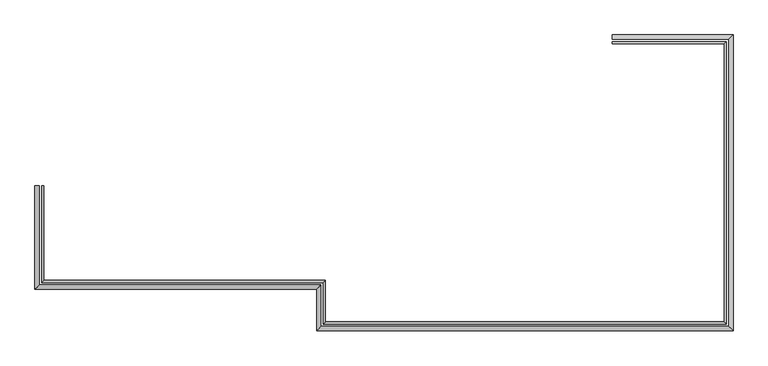
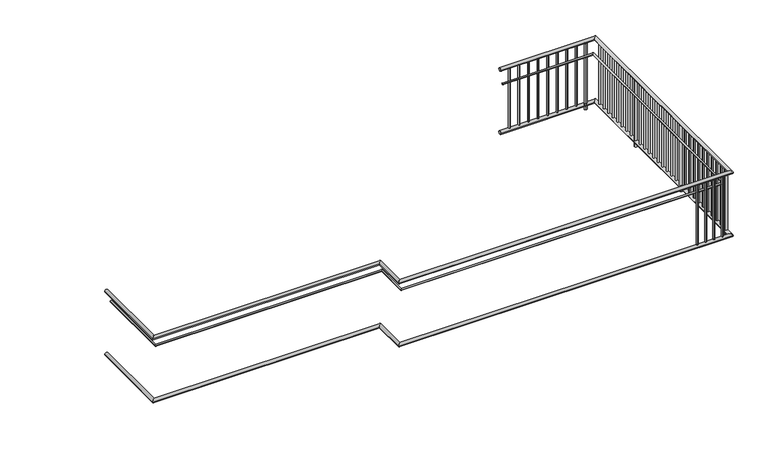
"""IFC4 building model written with IfcOpenShell, lengths in millimetres: railing geometry."""

from ifc_helpers import new_model, si_unit, point, frame, frame_2d, origin, place, context, project, spatial, circle_curve, ellipse_curve, trimmed, segment, composite_curve, outline, extrude, source, transform, mapped, element, save
from ifc_brep_helpers import plane_surface, cylinder_surface, advanced_brep


def railing_80b2a91e(model_context):
    return source(origin(), model_context, "Body", "SolidModel", [
        advanced_brep(
        [(-3300.274449, -6943.3965465, 4474.6), (-3249.474449, -6943.3965465, 4474.6), (-3249.474449, -8138.3965465, 4474.6), (-3300.274449, -8189.1965465, 4474.6), (144.725551, -8138.3965465, 4474.6), (93.925551, -8189.1965465, 4474.6), (144.725551, -8638.3965465, 4474.6), (93.925551, -8689.1965465, 4474.6), (5057.425551, -8638.3965465, 4474.6), (5108.225551, -8689.1965465, 4474.6), (5057.425551, -5178.2252792, 4474.6), (5108.225551, -5127.4252792, 4474.6), (3654.725551, -5127.4252792, 4474.6), (3654.725551, -5178.2252792, 4474.6)],
        [
            (0, 1, circle_curve(frame((-3274.874449, -6943.3965465, 4474.6), z_axis=(0.0, 1.0, 0.0), x_axis=(1.0, 0.0, 0.0)), 25.4)),
            (1, 0, circle_curve(frame((-3274.874449, -6943.3965465, 4474.6), z_axis=(0.0, 1.0, 0.0), x_axis=(1.0, 0.0, 0.0)), 25.4)),
            (1, 2),
            (2, 3, ellipse_curve(frame((-3274.874449, -8163.7965465, 4474.6), z_axis=(-0.7071067811865475, 0.7071067811865475, 0.0), x_axis=(0.7071067811865474, 0.7071067811865476, 0.0)), 35.9210245, 25.4)),
            (3, 0),
            (3, 2, ellipse_curve(frame((-3274.874449, -8163.7965465, 4474.6), z_axis=(-0.7071067811865475, 0.7071067811865475, 0.0), x_axis=(0.7071067811865474, 0.7071067811865476, 0.0)), 35.9210245, 25.4)),
            (2, 4),
            (4, 5, ellipse_curve(frame((119.325551, -8163.7965465, 4474.6), z_axis=(-0.7071067811865475, 0.7071067811865475, 0.0), x_axis=(-0.7071067811865476, -0.7071067811865474, 0.0)), 35.9210245, 25.4)),
            (5, 3),
            (5, 4, ellipse_curve(frame((119.325551, -8163.7965465, 4474.6), z_axis=(-0.7071067811865475, 0.7071067811865475, 0.0), x_axis=(-0.7071067811865476, -0.7071067811865474, 0.0)), 35.9210245, 25.4)),
            (4, 6),
            (6, 7, ellipse_curve(frame((119.325551, -8663.7965465, 4474.6), z_axis=(-0.7071067811865475, 0.7071067811865475, 0.0), x_axis=(0.7071067811865474, 0.7071067811865476, 0.0)), 35.9210245, 25.4)),
            (7, 5),
            (7, 6, ellipse_curve(frame((119.325551, -8663.7965465, 4474.6), z_axis=(-0.7071067811865475, 0.7071067811865475, 0.0), x_axis=(0.7071067811865474, 0.7071067811865476, 0.0)), 35.9210245, 25.4)),
            (6, 8),
            (8, 9, ellipse_curve(frame((5082.825551, -8663.7965465, 4474.6), z_axis=(-0.7071067811865475, -0.7071067811865475, 0.0), x_axis=(-0.7071067811865476, 0.7071067811865474, 0.0)), 35.9210245, 25.4)),
            (9, 7),
            (9, 8, ellipse_curve(frame((5082.825551, -8663.7965465, 4474.6), z_axis=(-0.7071067811865475, -0.7071067811865475, 0.0), x_axis=(-0.7071067811865476, 0.7071067811865474, 0.0)), 35.9210245, 25.4)),
            (8, 10),
            (10, 11, ellipse_curve(frame((5082.825551, -5152.8252792, 4474.6), z_axis=(0.7071067811865475, -0.7071067811865475, 0.0), x_axis=(-0.7071067811865474, -0.7071067811865476, 0.0)), 35.9210245, 25.4)),
            (11, 9),
            (11, 10, ellipse_curve(frame((5082.825551, -5152.8252792, 4474.6), z_axis=(0.7071067811865475, -0.7071067811865475, 0.0), x_axis=(-0.7071067811865474, -0.7071067811865476, 0.0)), 35.9210245, 25.4)),
            (12, 13, circle_curve(frame((3654.725551, -5152.8252792, 4474.6), z_axis=(-1.0, 0.0, 0.0), x_axis=(0.0, -1.0, 0.0)), 25.4)),
            (13, 12, circle_curve(frame((3654.725551, -5152.8252792, 4474.6), z_axis=(-1.0, 0.0, 0.0), x_axis=(0.0, -1.0, 0.0)), 25.4)),
            (10, 13),
            (12, 11),
        ],
        [
            plane_surface(frame((-3274.874449, -6943.3965465, 4500.0), z_axis=(0.0, 1.0, 0.0), x_axis=(0.0, 0.0, -1.0))),
            cylinder_surface(frame((-3274.874449, -6943.3965465, 4474.6), z_axis=(0.0, 1.0, 0.0), x_axis=(1.0, 0.0, 0.0)), 25.4),
            cylinder_surface(frame((-3274.874449, -8163.7965465, 4474.6), z_axis=(-1.0, 0.0, 0.0), x_axis=(0.0, 1.0, 0.0)), 25.4),
            cylinder_surface(frame((119.325551, -8163.7965465, 4474.6), z_axis=(0.0, 1.0, 0.0), x_axis=(1.0, 0.0, 0.0)), 25.4),
            cylinder_surface(frame((119.325551, -8663.7965465, 4474.6), z_axis=(-1.0, 0.0, 0.0), x_axis=(0.0, 1.0, 0.0)), 25.4),
            cylinder_surface(frame((5082.825551, -8663.7965465, 4474.6), z_axis=(0.0, -1.0, 0.0), x_axis=(-1.0, 0.0, 0.0)), 25.4),
            plane_surface(frame((3654.725551, -5152.8252792, 4500.0), z_axis=(-1.0, 0.0, 0.0), x_axis=(0.0, -1.0, 0.0))),
            cylinder_surface(frame((5082.825551, -5152.8252792, 4474.6), z_axis=(1.0, 0.0, 0.0), x_axis=(0.0, -1.0, 0.0)), 25.4),
        ],
        [
            (0, [[1, 2]]),
            (1, [[-2, 3, 4, 5]]),
            (1, [[-1, -5, 6, -3]]),
            (2, [[-4, 7, 8, 9]]),
            (2, [[-6, -9, 10, -7]]),
            (3, [[-8, 11, 12, 13]]),
            (3, [[-10, -13, 14, -11]]),
            (4, [[-12, 15, 16, 17]]),
            (4, [[-14, -17, 18, -15]]),
            (5, [[-16, 19, 20, 21]]),
            (5, [[-18, -21, 22, -19]]),
            (6, [[23, 24]]),
            (7, [[-20, 25, -23, 26]]),
            (7, [[-22, -26, -24, -25]]),
        ],
    ),
        advanced_brep(
        [(-3220.574449, -6943.3965465, 4287.3), (-3195.174449, -6943.3965465, 4287.3), (-3195.174449, -8084.0965465, 4287.3), (-3220.574449, -8109.4965465, 4287.3), (199.025551, -8084.0965465, 4287.3), (173.625551, -8109.4965465, 4287.3), (199.025551, -8584.0965465, 4287.3), (173.625551, -8609.4965465, 4287.3), (5003.125551, -8584.0965465, 4287.3), (5028.525551, -8609.4965465, 4287.3), (5003.125551, -5232.5252792, 4287.3), (5028.525551, -5207.1252792, 4287.3), (3654.725551, -5207.1252792, 4287.3), (3654.725551, -5232.5252792, 4287.3)],
        [
            (0, 1, circle_curve(frame((-3207.874449, -6943.3965465, 4287.3), z_axis=(0.0, 1.0, 0.0), x_axis=(1.0, 0.0, 0.0)), 12.7)),
            (1, 0, circle_curve(frame((-3207.874449, -6943.3965465, 4287.3), z_axis=(0.0, 1.0, 0.0), x_axis=(1.0, 0.0, 0.0)), 12.7)),
            (1, 2),
            (2, 3, ellipse_curve(frame((-3207.874449, -8096.7965465, 4287.3), z_axis=(-0.7071067811865475, 0.7071067811865475, 0.0), x_axis=(0.7071067811865474, 0.7071067811865476, 0.0)), 17.9605122, 12.7)),
            (3, 0),
            (3, 2, ellipse_curve(frame((-3207.874449, -8096.7965465, 4287.3), z_axis=(-0.7071067811865475, 0.7071067811865475, 0.0), x_axis=(0.7071067811865474, 0.7071067811865476, 0.0)), 17.9605122, 12.7)),
            (2, 4),
            (4, 5, ellipse_curve(frame((186.325551, -8096.7965465, 4287.3), z_axis=(-0.7071067811865475, 0.7071067811865475, 0.0), x_axis=(-0.7071067811865476, -0.7071067811865474, 0.0)), 17.9605122, 12.7)),
            (5, 3),
            (5, 4, ellipse_curve(frame((186.325551, -8096.7965465, 4287.3), z_axis=(-0.7071067811865475, 0.7071067811865475, 0.0), x_axis=(-0.7071067811865476, -0.7071067811865474, 0.0)), 17.9605122, 12.7)),
            (4, 6),
            (6, 7, ellipse_curve(frame((186.325551, -8596.7965465, 4287.3), z_axis=(-0.7071067811865475, 0.7071067811865475, 0.0), x_axis=(0.7071067811865474, 0.7071067811865476, 0.0)), 17.9605122, 12.7)),
            (7, 5),
            (7, 6, ellipse_curve(frame((186.325551, -8596.7965465, 4287.3), z_axis=(-0.7071067811865475, 0.7071067811865475, 0.0), x_axis=(0.7071067811865474, 0.7071067811865476, 0.0)), 17.9605122, 12.7)),
            (6, 8),
            (8, 9, ellipse_curve(frame((5015.825551, -8596.7965465, 4287.3), z_axis=(-0.7071067811865475, -0.7071067811865475, 0.0), x_axis=(-0.7071067811865476, 0.7071067811865474, 0.0)), 17.9605122, 12.7)),
            (9, 7),
            (9, 8, ellipse_curve(frame((5015.825551, -8596.7965465, 4287.3), z_axis=(-0.7071067811865475, -0.7071067811865475, 0.0), x_axis=(-0.7071067811865476, 0.7071067811865474, 0.0)), 17.9605122, 12.7)),
            (8, 10),
            (10, 11, ellipse_curve(frame((5015.825551, -5219.8252792, 4287.3), z_axis=(0.7071067811865475, -0.7071067811865475, 0.0), x_axis=(-0.7071067811865474, -0.7071067811865476, 0.0)), 17.9605122, 12.7)),
            (11, 9),
            (11, 10, ellipse_curve(frame((5015.825551, -5219.8252792, 4287.3), z_axis=(0.7071067811865475, -0.7071067811865475, 0.0), x_axis=(-0.7071067811865474, -0.7071067811865476, 0.0)), 17.9605122, 12.7)),
            (12, 13, circle_curve(frame((3654.725551, -5219.8252792, 4287.3), z_axis=(-1.0, 0.0, 0.0), x_axis=(0.0, -1.0, 0.0)), 12.7)),
            (13, 12, circle_curve(frame((3654.725551, -5219.8252792, 4287.3), z_axis=(-1.0, 0.0, 0.0), x_axis=(0.0, -1.0, 0.0)), 12.7)),
            (10, 13),
            (12, 11),
        ],
        [
            plane_surface(frame((-3207.874449, -6943.3965465, 4300.0), z_axis=(0.0, 1.0, 0.0), x_axis=(0.0, 0.0, -1.0))),
            cylinder_surface(frame((-3207.874449, -6943.3965465, 4287.3), z_axis=(0.0, 1.0, 0.0), x_axis=(1.0, 0.0, 0.0)), 12.7),
            cylinder_surface(frame((-3207.874449, -8096.7965465, 4287.3), z_axis=(-1.0, 0.0, 0.0), x_axis=(0.0, 1.0, 0.0)), 12.7),
            cylinder_surface(frame((186.325551, -8096.7965465, 4287.3), z_axis=(0.0, 1.0, 0.0), x_axis=(1.0, 0.0, 0.0)), 12.7),
            cylinder_surface(frame((186.325551, -8596.7965465, 4287.3), z_axis=(-1.0, 0.0, 0.0), x_axis=(0.0, 1.0, 0.0)), 12.7),
            cylinder_surface(frame((5015.825551, -8596.7965465, 4287.3), z_axis=(0.0, -1.0, 0.0), x_axis=(-1.0, 0.0, 0.0)), 12.7),
            plane_surface(frame((3654.725551, -5219.8252792, 4300.0), z_axis=(-1.0, 0.0, 0.0), x_axis=(0.0, -1.0, 0.0))),
            cylinder_surface(frame((5015.825551, -5219.8252792, 4287.3), z_axis=(1.0, 0.0, 0.0), x_axis=(0.0, -1.0, 0.0)), 12.7),
        ],
        [
            (0, [[1, 2]]),
            (1, [[-2, 3, 4, 5]]),
            (1, [[-1, -5, 6, -3]]),
            (2, [[-4, 7, 8, 9]]),
            (2, [[-6, -9, 10, -7]]),
            (3, [[-8, 11, 12, 13]]),
            (3, [[-10, -13, 14, -11]]),
            (4, [[-12, 15, 16, 17]]),
            (4, [[-14, -17, 18, -15]]),
            (5, [[-16, 19, 20, 21]]),
            (5, [[-18, -21, 22, -19]]),
            (6, [[23, 24]]),
            (7, [[-20, 25, -23, 26]]),
            (7, [[-22, -26, -24, -25]]),
        ],
    ),
        advanced_brep(
        [(-3300.274449, -6943.3965465, 3474.6), (-3249.474449, -6943.3965465, 3474.6), (-3249.474449, -8138.3965465, 3474.6), (-3300.274449, -8189.1965465, 3474.6), (144.725551, -8138.3965465, 3474.6), (93.925551, -8189.1965465, 3474.6), (144.725551, -8638.3965465, 3474.6), (93.925551, -8689.1965465, 3474.6), (5057.425551, -8638.3965465, 3474.6), (5108.225551, -8689.1965465, 3474.6), (5057.425551, -5178.2252792, 3474.6), (5108.225551, -5127.4252792, 3474.6), (3654.725551, -5127.4252792, 3474.6), (3654.725551, -5178.2252792, 3474.6)],
        [
            (0, 1, circle_curve(frame((-3274.874449, -6943.3965465, 3474.6), z_axis=(0.0, 1.0, 0.0), x_axis=(1.0, 0.0, 0.0)), 25.4)),
            (1, 0, circle_curve(frame((-3274.874449, -6943.3965465, 3474.6), z_axis=(0.0, 1.0, 0.0), x_axis=(1.0, 0.0, 0.0)), 25.4)),
            (1, 2),
            (2, 3, ellipse_curve(frame((-3274.874449, -8163.7965465, 3474.6), z_axis=(-0.7071067811865475, 0.7071067811865475, 0.0), x_axis=(0.7071067811865474, 0.7071067811865476, 0.0)), 35.9210245, 25.4)),
            (3, 0),
            (3, 2, ellipse_curve(frame((-3274.874449, -8163.7965465, 3474.6), z_axis=(-0.7071067811865475, 0.7071067811865475, 0.0), x_axis=(0.7071067811865474, 0.7071067811865476, 0.0)), 35.9210245, 25.4)),
            (2, 4),
            (4, 5, ellipse_curve(frame((119.325551, -8163.7965465, 3474.6), z_axis=(-0.7071067811865475, 0.7071067811865475, 0.0), x_axis=(-0.7071067811865476, -0.7071067811865474, 0.0)), 35.9210245, 25.4)),
            (5, 3),
            (5, 4, ellipse_curve(frame((119.325551, -8163.7965465, 3474.6), z_axis=(-0.7071067811865475, 0.7071067811865475, 0.0), x_axis=(-0.7071067811865476, -0.7071067811865474, 0.0)), 35.9210245, 25.4)),
            (4, 6),
            (6, 7, ellipse_curve(frame((119.325551, -8663.7965465, 3474.6), z_axis=(-0.7071067811865475, 0.7071067811865475, 0.0), x_axis=(0.7071067811865474, 0.7071067811865476, 0.0)), 35.9210245, 25.4)),
            (7, 5),
            (7, 6, ellipse_curve(frame((119.325551, -8663.7965465, 3474.6), z_axis=(-0.7071067811865475, 0.7071067811865475, 0.0), x_axis=(0.7071067811865474, 0.7071067811865476, 0.0)), 35.9210245, 25.4)),
            (6, 8),
            (8, 9, ellipse_curve(frame((5082.825551, -8663.7965465, 3474.6), z_axis=(-0.7071067811865475, -0.7071067811865475, 0.0), x_axis=(-0.7071067811865476, 0.7071067811865474, 0.0)), 35.9210245, 25.4)),
            (9, 7),
            (9, 8, ellipse_curve(frame((5082.825551, -8663.7965465, 3474.6), z_axis=(-0.7071067811865475, -0.7071067811865475, 0.0), x_axis=(-0.7071067811865476, 0.7071067811865474, 0.0)), 35.9210245, 25.4)),
            (8, 10),
            (10, 11, ellipse_curve(frame((5082.825551, -5152.8252792, 3474.6), z_axis=(0.7071067811865475, -0.7071067811865475, 0.0), x_axis=(-0.7071067811865474, -0.7071067811865476, 0.0)), 35.9210245, 25.4)),
            (11, 9),
            (11, 10, ellipse_curve(frame((5082.825551, -5152.8252792, 3474.6), z_axis=(0.7071067811865475, -0.7071067811865475, 0.0), x_axis=(-0.7071067811865474, -0.7071067811865476, 0.0)), 35.9210245, 25.4)),
            (12, 13, circle_curve(frame((3654.725551, -5152.8252792, 3474.6), z_axis=(-1.0, 0.0, 0.0), x_axis=(0.0, -1.0, 0.0)), 25.4)),
            (13, 12, circle_curve(frame((3654.725551, -5152.8252792, 3474.6), z_axis=(-1.0, 0.0, 0.0), x_axis=(0.0, -1.0, 0.0)), 25.4)),
            (10, 13),
            (12, 11),
        ],
        [
            plane_surface(frame((-3274.874449, -6943.3965465, 3500.0), z_axis=(0.0, 1.0, 0.0), x_axis=(0.0, 0.0, -1.0))),
            cylinder_surface(frame((-3274.874449, -6943.3965465, 3474.6), z_axis=(0.0, 1.0, 0.0), x_axis=(1.0, 0.0, 0.0)), 25.4),
            cylinder_surface(frame((-3274.874449, -8163.7965465, 3474.6), z_axis=(-1.0, 0.0, 0.0), x_axis=(0.0, 1.0, 0.0)), 25.4),
            cylinder_surface(frame((119.325551, -8163.7965465, 3474.6), z_axis=(0.0, 1.0, 0.0), x_axis=(1.0, 0.0, 0.0)), 25.4),
            cylinder_surface(frame((119.325551, -8663.7965465, 3474.6), z_axis=(-1.0, 0.0, 0.0), x_axis=(0.0, 1.0, 0.0)), 25.4),
            cylinder_surface(frame((5082.825551, -8663.7965465, 3474.6), z_axis=(0.0, -1.0, 0.0), x_axis=(-1.0, 0.0, 0.0)), 25.4),
            plane_surface(frame((3654.725551, -5152.8252792, 3500.0), z_axis=(-1.0, 0.0, 0.0), x_axis=(0.0, -1.0, 0.0))),
            cylinder_surface(frame((5082.825551, -5152.8252792, 3474.6), z_axis=(1.0, 0.0, 0.0), x_axis=(0.0, -1.0, 0.0)), 25.4),
        ],
        [
            (0, [[1, 2]]),
            (1, [[-2, 3, 4, 5]]),
            (1, [[-1, -5, 6, -3]]),
            (2, [[-4, 7, 8, 9]]),
            (2, [[-6, -9, 10, -7]]),
            (3, [[-8, 11, 12, 13]]),
            (3, [[-10, -13, 14, -11]]),
            (4, [[-12, 15, 16, 17]]),
            (4, [[-14, -17, 18, -15]]),
            (5, [[-16, 19, 20, 21]]),
            (5, [[-18, -21, 22, -19]]),
            (6, [[23, 24]]),
            (7, [[-20, 25, -23, 26]]),
            (7, [[-22, -26, -24, -25]]),
        ],
    ),
        extrude(outline(composite_curve([segment(trimmed(circle_curve(frame_2d((3797.535551, -5152.8252792)), 12.5), [point((3797.535551, -5140.3252792))], [point((3797.535551, -5165.3252792))], False, "CARTESIAN"), True, "CONTINUOUS"), segment(trimmed(circle_curve(frame_2d((3797.535551, -5152.8252792)), 12.5), [point((3797.535551, -5165.3252792))], [point((3797.535551, -5140.3252792))], False, "CARTESIAN"), True, "CONTINUOUS")], self_intersect=False)), frame((0.0, 0.0, 3500.0), z_axis=(0.0, 0.0, 1.0), x_axis=(1.0, 0.0, 0.0)), (0.0, 0.0, 1.0), 949.2),
        extrude(outline(composite_curve([segment(trimmed(circle_curve(frame_2d((3940.345551, -5152.8252792)), 12.5), [point((3940.345551, -5140.3252792))], [point((3940.345551, -5165.3252792))], False, "CARTESIAN"), True, "CONTINUOUS"), segment(trimmed(circle_curve(frame_2d((3940.345551, -5152.8252792)), 12.5), [point((3940.345551, -5165.3252792))], [point((3940.345551, -5140.3252792))], False, "CARTESIAN"), True, "CONTINUOUS")], self_intersect=False)), frame((0.0, 0.0, 3500.0), z_axis=(0.0, 0.0, 1.0), x_axis=(1.0, 0.0, 0.0)), (0.0, 0.0, 1.0), 949.2),
        extrude(outline(composite_curve([segment(trimmed(circle_curve(frame_2d((4083.155551, -5152.8252792)), 12.5), [point((4083.155551, -5140.3252792))], [point((4083.155551, -5165.3252792))], False, "CARTESIAN"), True, "CONTINUOUS"), segment(trimmed(circle_curve(frame_2d((4083.155551, -5152.8252792)), 12.5), [point((4083.155551, -5165.3252792))], [point((4083.155551, -5140.3252792))], False, "CARTESIAN"), True, "CONTINUOUS")], self_intersect=False)), frame((0.0, 0.0, 3500.0), z_axis=(0.0, 0.0, 1.0), x_axis=(1.0, 0.0, 0.0)), (0.0, 0.0, 1.0), 949.2),
        extrude(outline(composite_curve([segment(trimmed(circle_curve(frame_2d((4225.965551, -5152.8252792)), 12.5), [point((4225.965551, -5140.3252792))], [point((4225.965551, -5165.3252792))], False, "CARTESIAN"), True, "CONTINUOUS"), segment(trimmed(circle_curve(frame_2d((4225.965551, -5152.8252792)), 12.5), [point((4225.965551, -5165.3252792))], [point((4225.965551, -5140.3252792))], False, "CARTESIAN"), True, "CONTINUOUS")], self_intersect=False)), frame((0.0, 0.0, 3500.0), z_axis=(0.0, 0.0, 1.0), x_axis=(1.0, 0.0, 0.0)), (0.0, 0.0, 1.0), 949.2),
        extrude(outline(composite_curve([segment(trimmed(circle_curve(frame_2d((4368.775551, -5152.8252792)), 12.5), [point((4368.775551, -5140.3252792))], [point((4368.775551, -5165.3252792))], False, "CARTESIAN"), True, "CONTINUOUS"), segment(trimmed(circle_curve(frame_2d((4368.775551, -5152.8252792)), 12.5), [point((4368.775551, -5165.3252792))], [point((4368.775551, -5140.3252792))], False, "CARTESIAN"), True, "CONTINUOUS")], self_intersect=False)), frame((0.0, 0.0, 3500.0), z_axis=(0.0, 0.0, 1.0), x_axis=(1.0, 0.0, 0.0)), (0.0, 0.0, 1.0), 949.2),
        extrude(outline(composite_curve([segment(trimmed(circle_curve(frame_2d((4511.585551, -5152.8252792)), 12.5), [point((4511.585551, -5140.3252792))], [point((4511.585551, -5165.3252792))], False, "CARTESIAN"), True, "CONTINUOUS"), segment(trimmed(circle_curve(frame_2d((4511.585551, -5152.8252792)), 12.5), [point((4511.585551, -5165.3252792))], [point((4511.585551, -5140.3252792))], False, "CARTESIAN"), True, "CONTINUOUS")], self_intersect=False)), frame((0.0, 0.0, 3500.0), z_axis=(0.0, 0.0, 1.0), x_axis=(1.0, 0.0, 0.0)), (0.0, 0.0, 1.0), 949.2),
        extrude(outline(composite_curve([segment(trimmed(circle_curve(frame_2d((4654.395551, -5152.8252792)), 12.5), [point((4654.395551, -5140.3252792))], [point((4654.395551, -5165.3252792))], False, "CARTESIAN"), True, "CONTINUOUS"), segment(trimmed(circle_curve(frame_2d((4654.395551, -5152.8252792)), 12.5), [point((4654.395551, -5165.3252792))], [point((4654.395551, -5140.3252792))], False, "CARTESIAN"), True, "CONTINUOUS")], self_intersect=False)), frame((0.0, 0.0, 3500.0), z_axis=(0.0, 0.0, 1.0), x_axis=(1.0, 0.0, 0.0)), (0.0, 0.0, 1.0), 949.2),
        extrude(outline(composite_curve([segment(trimmed(circle_curve(frame_2d((4797.205551, -5152.8252792)), 12.5), [point((4797.205551, -5140.3252792))], [point((4797.205551, -5165.3252792))], False, "CARTESIAN"), True, "CONTINUOUS"), segment(trimmed(circle_curve(frame_2d((4797.205551, -5152.8252792)), 12.5), [point((4797.205551, -5165.3252792))], [point((4797.205551, -5140.3252792))], False, "CARTESIAN"), True, "CONTINUOUS")], self_intersect=False)), frame((0.0, 0.0, 3500.0), z_axis=(0.0, 0.0, 1.0), x_axis=(1.0, 0.0, 0.0)), (0.0, 0.0, 1.0), 949.2),
        extrude(outline(composite_curve([segment(trimmed(circle_curve(frame_2d((4940.015551, -5152.8252792)), 21.0), [point((4940.015551, -5131.8252792))], [point((4940.015551, -5173.8252792))], False, "CARTESIAN"), True, "CONTINUOUS"), segment(trimmed(circle_curve(frame_2d((4940.015551, -5152.8252792)), 21.0), [point((4940.015551, -5173.8252792))], [point((4940.015551, -5131.8252792))], False, "CARTESIAN"), True, "CONTINUOUS")], self_intersect=False)), frame((0.0, 0.0, 3400.0), z_axis=(0.0, 0.0, 1.0), x_axis=(1.0, 0.0, 0.0)), (0.0, 0.0, 1.0), 1049.2),
        extrude(outline(composite_curve([segment(trimmed(circle_curve(frame_2d((5082.825551, -5269.8576547)), 12.5), [point((5095.325551, -5269.8576547))], [point((5070.325551, -5269.8576547))], False, "CARTESIAN"), True, "CONTINUOUS"), segment(trimmed(circle_curve(frame_2d((5082.825551, -5269.8576547)), 12.5), [point((5070.325551, -5269.8576547))], [point((5095.325551, -5269.8576547))], False, "CARTESIAN"), True, "CONTINUOUS")], self_intersect=False)), frame((0.0, 0.0, 3500.0), z_axis=(0.0, 0.0, 1.0), x_axis=(1.0, 0.0, 0.0)), (0.0, 0.0, 1.0), 949.2),
        extrude(outline(composite_curve([segment(trimmed(circle_curve(frame_2d((5082.825551, -5386.8900303)), 12.5), [point((5095.325551, -5386.8900303))], [point((5070.325551, -5386.8900303))], False, "CARTESIAN"), True, "CONTINUOUS"), segment(trimmed(circle_curve(frame_2d((5082.825551, -5386.8900303)), 12.5), [point((5070.325551, -5386.8900303))], [point((5095.325551, -5386.8900303))], False, "CARTESIAN"), True, "CONTINUOUS")], self_intersect=False)), frame((0.0, 0.0, 3500.0), z_axis=(0.0, 0.0, 1.0), x_axis=(1.0, 0.0, 0.0)), (0.0, 0.0, 1.0), 949.2),
        extrude(outline(composite_curve([segment(trimmed(circle_curve(frame_2d((5082.825551, -5503.9224059)), 12.5), [point((5095.325551, -5503.9224059))], [point((5070.325551, -5503.9224059))], False, "CARTESIAN"), True, "CONTINUOUS"), segment(trimmed(circle_curve(frame_2d((5082.825551, -5503.9224059)), 12.5), [point((5070.325551, -5503.9224059))], [point((5095.325551, -5503.9224059))], False, "CARTESIAN"), True, "CONTINUOUS")], self_intersect=False)), frame((0.0, 0.0, 3500.0), z_axis=(0.0, 0.0, 1.0), x_axis=(1.0, 0.0, 0.0)), (0.0, 0.0, 1.0), 949.2),
        extrude(outline(composite_curve([segment(trimmed(circle_curve(frame_2d((5082.825551, -5620.9547815)), 12.5), [point((5095.325551, -5620.9547815))], [point((5070.325551, -5620.9547815))], False, "CARTESIAN"), True, "CONTINUOUS"), segment(trimmed(circle_curve(frame_2d((5082.825551, -5620.9547815)), 12.5), [point((5070.325551, -5620.9547815))], [point((5095.325551, -5620.9547815))], False, "CARTESIAN"), True, "CONTINUOUS")], self_intersect=False)), frame((0.0, 0.0, 3500.0), z_axis=(0.0, 0.0, 1.0), x_axis=(1.0, 0.0, 0.0)), (0.0, 0.0, 1.0), 949.2),
        extrude(outline(composite_curve([segment(trimmed(circle_curve(frame_2d((5082.825551, -5737.9871571)), 12.5), [point((5095.325551, -5737.9871571))], [point((5070.325551, -5737.9871571))], False, "CARTESIAN"), True, "CONTINUOUS"), segment(trimmed(circle_curve(frame_2d((5082.825551, -5737.9871571)), 12.5), [point((5070.325551, -5737.9871571))], [point((5095.325551, -5737.9871571))], False, "CARTESIAN"), True, "CONTINUOUS")], self_intersect=False)), frame((0.0, 0.0, 3500.0), z_axis=(0.0, 0.0, 1.0), x_axis=(1.0, 0.0, 0.0)), (0.0, 0.0, 1.0), 949.2),
        extrude(outline(composite_curve([segment(trimmed(circle_curve(frame_2d((5082.825551, -5855.0195326)), 12.5), [point((5095.325551, -5855.0195326))], [point((5070.325551, -5855.0195326))], False, "CARTESIAN"), True, "CONTINUOUS"), segment(trimmed(circle_curve(frame_2d((5082.825551, -5855.0195326)), 12.5), [point((5070.325551, -5855.0195326))], [point((5095.325551, -5855.0195326))], False, "CARTESIAN"), True, "CONTINUOUS")], self_intersect=False)), frame((0.0, 0.0, 3500.0), z_axis=(0.0, 0.0, 1.0), x_axis=(1.0, 0.0, 0.0)), (0.0, 0.0, 1.0), 949.2),
        extrude(outline(composite_curve([segment(trimmed(circle_curve(frame_2d((5082.825551, -5972.0519082)), 12.5), [point((5095.325551, -5972.0519082))], [point((5070.325551, -5972.0519082))], False, "CARTESIAN"), True, "CONTINUOUS"), segment(trimmed(circle_curve(frame_2d((5082.825551, -5972.0519082)), 12.5), [point((5070.325551, -5972.0519082))], [point((5095.325551, -5972.0519082))], False, "CARTESIAN"), True, "CONTINUOUS")], self_intersect=False)), frame((0.0, 0.0, 3500.0), z_axis=(0.0, 0.0, 1.0), x_axis=(1.0, 0.0, 0.0)), (0.0, 0.0, 1.0), 949.2),
        extrude(outline(composite_curve([segment(trimmed(circle_curve(frame_2d((5082.825551, -6089.0842838)), 12.5), [point((5095.325551, -6089.0842838))], [point((5070.325551, -6089.0842838))], False, "CARTESIAN"), True, "CONTINUOUS"), segment(trimmed(circle_curve(frame_2d((5082.825551, -6089.0842838)), 12.5), [point((5070.325551, -6089.0842838))], [point((5095.325551, -6089.0842838))], False, "CARTESIAN"), True, "CONTINUOUS")], self_intersect=False)), frame((0.0, 0.0, 3500.0), z_axis=(0.0, 0.0, 1.0), x_axis=(1.0, 0.0, 0.0)), (0.0, 0.0, 1.0), 949.2),
        extrude(outline(composite_curve([segment(trimmed(circle_curve(frame_2d((5082.825551, -6206.1166594)), 21.0), [point((5103.825551, -6206.1166594))], [point((5061.825551, -6206.1166594))], False, "CARTESIAN"), True, "CONTINUOUS"), segment(trimmed(circle_curve(frame_2d((5082.825551, -6206.1166594)), 21.0), [point((5061.825551, -6206.1166594))], [point((5103.825551, -6206.1166594))], False, "CARTESIAN"), True, "CONTINUOUS")], self_intersect=False)), frame((0.0, 0.0, 3400.0), z_axis=(0.0, 0.0, 1.0), x_axis=(1.0, 0.0, 0.0)), (0.0, 0.0, 1.0), 1049.2),
        extrude(outline(composite_curve([segment(trimmed(circle_curve(frame_2d((5082.825551, -6323.1490349)), 12.5), [point((5095.325551, -6323.1490349))], [point((5070.325551, -6323.1490349))], False, "CARTESIAN"), True, "CONTINUOUS"), segment(trimmed(circle_curve(frame_2d((5082.825551, -6323.1490349)), 12.5), [point((5070.325551, -6323.1490349))], [point((5095.325551, -6323.1490349))], False, "CARTESIAN"), True, "CONTINUOUS")], self_intersect=False)), frame((0.0, 0.0, 3500.0), z_axis=(0.0, 0.0, 1.0), x_axis=(1.0, 0.0, 0.0)), (0.0, 0.0, 1.0), 949.2),
        extrude(outline(composite_curve([segment(trimmed(circle_curve(frame_2d((5082.825551, -6440.1814105)), 12.5), [point((5095.325551, -6440.1814105))], [point((5070.325551, -6440.1814105))], False, "CARTESIAN"), True, "CONTINUOUS"), segment(trimmed(circle_curve(frame_2d((5082.825551, -6440.1814105)), 12.5), [point((5070.325551, -6440.1814105))], [point((5095.325551, -6440.1814105))], False, "CARTESIAN"), True, "CONTINUOUS")], self_intersect=False)), frame((0.0, 0.0, 3500.0), z_axis=(0.0, 0.0, 1.0), x_axis=(1.0, 0.0, 0.0)), (0.0, 0.0, 1.0), 949.2),
        extrude(outline(composite_curve([segment(trimmed(circle_curve(frame_2d((5082.825551, -6557.2137861)), 12.5), [point((5095.325551, -6557.2137861))], [point((5070.325551, -6557.2137861))], False, "CARTESIAN"), True, "CONTINUOUS"), segment(trimmed(circle_curve(frame_2d((5082.825551, -6557.2137861)), 12.5), [point((5070.325551, -6557.2137861))], [point((5095.325551, -6557.2137861))], False, "CARTESIAN"), True, "CONTINUOUS")], self_intersect=False)), frame((0.0, 0.0, 3500.0), z_axis=(0.0, 0.0, 1.0), x_axis=(1.0, 0.0, 0.0)), (0.0, 0.0, 1.0), 949.2),
        extrude(outline(composite_curve([segment(trimmed(circle_curve(frame_2d((5082.825551, -6674.2461617)), 12.5), [point((5095.325551, -6674.2461617))], [point((5070.325551, -6674.2461617))], False, "CARTESIAN"), True, "CONTINUOUS"), segment(trimmed(circle_curve(frame_2d((5082.825551, -6674.2461617)), 12.5), [point((5070.325551, -6674.2461617))], [point((5095.325551, -6674.2461617))], False, "CARTESIAN"), True, "CONTINUOUS")], self_intersect=False)), frame((0.0, 0.0, 3500.0), z_axis=(0.0, 0.0, 1.0), x_axis=(1.0, 0.0, 0.0)), (0.0, 0.0, 1.0), 949.2),
        extrude(outline(composite_curve([segment(trimmed(circle_curve(frame_2d((5082.825551, -6791.2785373)), 12.5), [point((5095.325551, -6791.2785373))], [point((5070.325551, -6791.2785373))], False, "CARTESIAN"), True, "CONTINUOUS"), segment(trimmed(circle_curve(frame_2d((5082.825551, -6791.2785373)), 12.5), [point((5070.325551, -6791.2785373))], [point((5095.325551, -6791.2785373))], False, "CARTESIAN"), True, "CONTINUOUS")], self_intersect=False)), frame((0.0, 0.0, 3500.0), z_axis=(0.0, 0.0, 1.0), x_axis=(1.0, 0.0, 0.0)), (0.0, 0.0, 1.0), 949.2),
        extrude(outline(composite_curve([segment(trimmed(circle_curve(frame_2d((5082.825551, -6908.3109128)), 12.5), [point((5095.325551, -6908.3109128))], [point((5070.325551, -6908.3109128))], False, "CARTESIAN"), True, "CONTINUOUS"), segment(trimmed(circle_curve(frame_2d((5082.825551, -6908.3109128)), 12.5), [point((5070.325551, -6908.3109128))], [point((5095.325551, -6908.3109128))], False, "CARTESIAN"), True, "CONTINUOUS")], self_intersect=False)), frame((0.0, 0.0, 3500.0), z_axis=(0.0, 0.0, 1.0), x_axis=(1.0, 0.0, 0.0)), (0.0, 0.0, 1.0), 949.2),
        extrude(outline(composite_curve([segment(trimmed(circle_curve(frame_2d((5082.825551, -7025.3432884)), 12.5), [point((5095.325551, -7025.3432884))], [point((5070.325551, -7025.3432884))], False, "CARTESIAN"), True, "CONTINUOUS"), segment(trimmed(circle_curve(frame_2d((5082.825551, -7025.3432884)), 12.5), [point((5070.325551, -7025.3432884))], [point((5095.325551, -7025.3432884))], False, "CARTESIAN"), True, "CONTINUOUS")], self_intersect=False)), frame((0.0, 0.0, 3500.0), z_axis=(0.0, 0.0, 1.0), x_axis=(1.0, 0.0, 0.0)), (0.0, 0.0, 1.0), 949.2),
        extrude(outline(composite_curve([segment(trimmed(circle_curve(frame_2d((5082.825551, -7142.375664)), 12.5), [point((5095.325551, -7142.375664))], [point((5070.325551, -7142.375664))], False, "CARTESIAN"), True, "CONTINUOUS"), segment(trimmed(circle_curve(frame_2d((5082.825551, -7142.375664)), 12.5), [point((5070.325551, -7142.375664))], [point((5095.325551, -7142.375664))], False, "CARTESIAN"), True, "CONTINUOUS")], self_intersect=False)), frame((0.0, 0.0, 3500.0), z_axis=(0.0, 0.0, 1.0), x_axis=(1.0, 0.0, 0.0)), (0.0, 0.0, 1.0), 949.2),
        extrude(outline(composite_curve([segment(trimmed(circle_curve(frame_2d((5082.825551, -7259.4080396)), 12.5), [point((5095.325551, -7259.4080396))], [point((5070.325551, -7259.4080396))], False, "CARTESIAN"), True, "CONTINUOUS"), segment(trimmed(circle_curve(frame_2d((5082.825551, -7259.4080396)), 12.5), [point((5070.325551, -7259.4080396))], [point((5095.325551, -7259.4080396))], False, "CARTESIAN"), True, "CONTINUOUS")], self_intersect=False)), frame((0.0, 0.0, 3500.0), z_axis=(0.0, 0.0, 1.0), x_axis=(1.0, 0.0, 0.0)), (0.0, 0.0, 1.0), 949.2),
        extrude(outline(composite_curve([segment(trimmed(circle_curve(frame_2d((5082.825551, -7376.4404152)), 21.0), [point((5103.825551, -7376.4404152))], [point((5061.825551, -7376.4404152))], False, "CARTESIAN"), True, "CONTINUOUS"), segment(trimmed(circle_curve(frame_2d((5082.825551, -7376.4404152)), 21.0), [point((5061.825551, -7376.4404152))], [point((5103.825551, -7376.4404152))], False, "CARTESIAN"), True, "CONTINUOUS")], self_intersect=False)), frame((0.0, 0.0, 3400.0), z_axis=(0.0, 0.0, 1.0), x_axis=(1.0, 0.0, 0.0)), (0.0, 0.0, 1.0), 1049.2),
        extrude(outline(composite_curve([segment(trimmed(circle_curve(frame_2d((5082.825551, -7493.4727907)), 12.5), [point((5095.325551, -7493.4727907))], [point((5070.325551, -7493.4727907))], False, "CARTESIAN"), True, "CONTINUOUS"), segment(trimmed(circle_curve(frame_2d((5082.825551, -7493.4727907)), 12.5), [point((5070.325551, -7493.4727907))], [point((5095.325551, -7493.4727907))], False, "CARTESIAN"), True, "CONTINUOUS")], self_intersect=False)), frame((0.0, 0.0, 3500.0), z_axis=(0.0, 0.0, 1.0), x_axis=(1.0, 0.0, 0.0)), (0.0, 0.0, 1.0), 949.2),
        extrude(outline(composite_curve([segment(trimmed(circle_curve(frame_2d((5082.825551, -7610.5051663)), 12.5), [point((5095.325551, -7610.5051663))], [point((5070.325551, -7610.5051663))], False, "CARTESIAN"), True, "CONTINUOUS"), segment(trimmed(circle_curve(frame_2d((5082.825551, -7610.5051663)), 12.5), [point((5070.325551, -7610.5051663))], [point((5095.325551, -7610.5051663))], False, "CARTESIAN"), True, "CONTINUOUS")], self_intersect=False)), frame((0.0, 0.0, 3500.0), z_axis=(0.0, 0.0, 1.0), x_axis=(1.0, 0.0, 0.0)), (0.0, 0.0, 1.0), 949.2),
        extrude(outline(composite_curve([segment(trimmed(circle_curve(frame_2d((5082.825551, -7727.5375419)), 12.5), [point((5095.325551, -7727.5375419))], [point((5070.325551, -7727.5375419))], False, "CARTESIAN"), True, "CONTINUOUS"), segment(trimmed(circle_curve(frame_2d((5082.825551, -7727.5375419)), 12.5), [point((5070.325551, -7727.5375419))], [point((5095.325551, -7727.5375419))], False, "CARTESIAN"), True, "CONTINUOUS")], self_intersect=False)), frame((0.0, 0.0, 3500.0), z_axis=(0.0, 0.0, 1.0), x_axis=(1.0, 0.0, 0.0)), (0.0, 0.0, 1.0), 949.2),
        extrude(outline(composite_curve([segment(trimmed(circle_curve(frame_2d((5082.825551, -7844.5699175)), 12.5), [point((5095.325551, -7844.5699175))], [point((5070.325551, -7844.5699175))], False, "CARTESIAN"), True, "CONTINUOUS"), segment(trimmed(circle_curve(frame_2d((5082.825551, -7844.5699175)), 12.5), [point((5070.325551, -7844.5699175))], [point((5095.325551, -7844.5699175))], False, "CARTESIAN"), True, "CONTINUOUS")], self_intersect=False)), frame((0.0, 0.0, 3500.0), z_axis=(0.0, 0.0, 1.0), x_axis=(1.0, 0.0, 0.0)), (0.0, 0.0, 1.0), 949.2),
        extrude(outline(composite_curve([segment(trimmed(circle_curve(frame_2d((5082.825551, -7961.6022931)), 12.5), [point((5095.325551, -7961.6022931))], [point((5070.325551, -7961.6022931))], False, "CARTESIAN"), True, "CONTINUOUS"), segment(trimmed(circle_curve(frame_2d((5082.825551, -7961.6022931)), 12.5), [point((5070.325551, -7961.6022931))], [point((5095.325551, -7961.6022931))], False, "CARTESIAN"), True, "CONTINUOUS")], self_intersect=False)), frame((0.0, 0.0, 3500.0), z_axis=(0.0, 0.0, 1.0), x_axis=(1.0, 0.0, 0.0)), (0.0, 0.0, 1.0), 949.2),
        extrude(outline(composite_curve([segment(trimmed(circle_curve(frame_2d((5082.825551, -8078.6346686)), 12.5), [point((5095.325551, -8078.6346686))], [point((5070.325551, -8078.6346686))], False, "CARTESIAN"), True, "CONTINUOUS"), segment(trimmed(circle_curve(frame_2d((5082.825551, -8078.6346686)), 12.5), [point((5070.325551, -8078.6346686))], [point((5095.325551, -8078.6346686))], False, "CARTESIAN"), True, "CONTINUOUS")], self_intersect=False)), frame((0.0, 0.0, 3500.0), z_axis=(0.0, 0.0, 1.0), x_axis=(1.0, 0.0, 0.0)), (0.0, 0.0, 1.0), 949.2),
        extrude(outline(composite_curve([segment(trimmed(circle_curve(frame_2d((5082.825551, -8195.6670442)), 12.5), [point((5095.325551, -8195.6670442))], [point((5070.325551, -8195.6670442))], False, "CARTESIAN"), True, "CONTINUOUS"), segment(trimmed(circle_curve(frame_2d((5082.825551, -8195.6670442)), 12.5), [point((5070.325551, -8195.6670442))], [point((5095.325551, -8195.6670442))], False, "CARTESIAN"), True, "CONTINUOUS")], self_intersect=False)), frame((0.0, 0.0, 3500.0), z_axis=(0.0, 0.0, 1.0), x_axis=(1.0, 0.0, 0.0)), (0.0, 0.0, 1.0), 949.2),
        extrude(outline(composite_curve([segment(trimmed(circle_curve(frame_2d((5082.825551, -8312.6994198)), 12.5), [point((5095.325551, -8312.6994198))], [point((5070.325551, -8312.6994198))], False, "CARTESIAN"), True, "CONTINUOUS"), segment(trimmed(circle_curve(frame_2d((5082.825551, -8312.6994198)), 12.5), [point((5070.325551, -8312.6994198))], [point((5095.325551, -8312.6994198))], False, "CARTESIAN"), True, "CONTINUOUS")], self_intersect=False)), frame((0.0, 0.0, 3500.0), z_axis=(0.0, 0.0, 1.0), x_axis=(1.0, 0.0, 0.0)), (0.0, 0.0, 1.0), 949.2),
        extrude(outline(composite_curve([segment(trimmed(circle_curve(frame_2d((5082.825551, -8429.7317954)), 12.5), [point((5095.325551, -8429.7317954))], [point((5070.325551, -8429.7317954))], False, "CARTESIAN"), True, "CONTINUOUS"), segment(trimmed(circle_curve(frame_2d((5082.825551, -8429.7317954)), 12.5), [point((5070.325551, -8429.7317954))], [point((5095.325551, -8429.7317954))], False, "CARTESIAN"), True, "CONTINUOUS")], self_intersect=False)), frame((0.0, 0.0, 3500.0), z_axis=(0.0, 0.0, 1.0), x_axis=(1.0, 0.0, 0.0)), (0.0, 0.0, 1.0), 949.2),
        extrude(outline(composite_curve([segment(trimmed(circle_curve(frame_2d((5082.825551, -8546.764171)), 21.0), [point((5103.825551, -8546.764171))], [point((5061.825551, -8546.764171))], False, "CARTESIAN"), True, "CONTINUOUS"), segment(trimmed(circle_curve(frame_2d((5082.825551, -8546.764171)), 21.0), [point((5061.825551, -8546.764171))], [point((5103.825551, -8546.764171))], False, "CARTESIAN"), True, "CONTINUOUS")], self_intersect=False)), frame((0.0, 0.0, 3400.0), z_axis=(0.0, 0.0, 1.0), x_axis=(1.0, 0.0, 0.0)), (0.0, 0.0, 1.0), 1049.2),
        extrude(outline(composite_curve([segment(trimmed(circle_curve(frame_2d((4958.738051, -8663.7965465)), 12.5), [point((4958.738051, -8676.2965465))], [point((4958.738051, -8651.2965465))], False, "CARTESIAN"), True, "CONTINUOUS"), segment(trimmed(circle_curve(frame_2d((4958.738051, -8663.7965465)), 12.5), [point((4958.738051, -8651.2965465))], [point((4958.738051, -8676.2965465))], False, "CARTESIAN"), True, "CONTINUOUS")], self_intersect=False)), frame((0.0, 0.0, 3500.0), z_axis=(0.0, 0.0, 1.0), x_axis=(1.0, 0.0, 0.0)), (0.0, 0.0, 1.0), 949.2),
        extrude(outline(composite_curve([segment(trimmed(circle_curve(frame_2d((4834.650551, -8663.7965465)), 12.5), [point((4834.650551, -8676.2965465))], [point((4834.650551, -8651.2965465))], False, "CARTESIAN"), True, "CONTINUOUS"), segment(trimmed(circle_curve(frame_2d((4834.650551, -8663.7965465)), 12.5), [point((4834.650551, -8651.2965465))], [point((4834.650551, -8676.2965465))], False, "CARTESIAN"), True, "CONTINUOUS")], self_intersect=False)), frame((0.0, 0.0, 3500.0), z_axis=(0.0, 0.0, 1.0), x_axis=(1.0, 0.0, 0.0)), (0.0, 0.0, 1.0), 949.2),
        extrude(outline(composite_curve([segment(trimmed(circle_curve(frame_2d((4710.563051, -8663.7965465)), 12.5), [point((4710.563051, -8676.2965465))], [point((4710.563051, -8651.2965465))], False, "CARTESIAN"), True, "CONTINUOUS"), segment(trimmed(circle_curve(frame_2d((4710.563051, -8663.7965465)), 12.5), [point((4710.563051, -8651.2965465))], [point((4710.563051, -8676.2965465))], False, "CARTESIAN"), True, "CONTINUOUS")], self_intersect=False)), frame((0.0, 0.0, 3500.0), z_axis=(0.0, 0.0, 1.0), x_axis=(1.0, 0.0, 0.0)), (0.0, 0.0, 1.0), 949.2),
        extrude(outline(composite_curve([segment(trimmed(circle_curve(frame_2d((4586.475551, -8663.7965465)), 12.5), [point((4586.475551, -8676.2965465))], [point((4586.475551, -8651.2965465))], False, "CARTESIAN"), True, "CONTINUOUS"), segment(trimmed(circle_curve(frame_2d((4586.475551, -8663.7965465)), 12.5), [point((4586.475551, -8651.2965465))], [point((4586.475551, -8676.2965465))], False, "CARTESIAN"), True, "CONTINUOUS")], self_intersect=False)), frame((0.0, 0.0, 3500.0), z_axis=(0.0, 0.0, 1.0), x_axis=(1.0, 0.0, 0.0)), (0.0, 0.0, 1.0), 949.2),
    ])


if __name__ == "__main__":
    model = new_model("IFC4")
    model_context = context("Model", 3, world=origin())
    ifc_project = project(units=[si_unit("LENGTHUNIT", "METRE", prefix="MILLI")], contexts=[model_context])
    site = spatial("IfcSite", under=ifc_project)
    building = spatial("IfcBuilding", under=site)
    placement = place(None, origin())
    railing_shape = railing_80b2a91e(model_context)
    element("IfcRailing", 1, at=placement, inside=building, context=model_context, shape_type="MappedRepresentation", body=[
        mapped(railing_shape, transform((0.0, 0.0, 0.0), x_axis=(1.0, 0.0, 0.0), y_axis=(0.0, 1.0, 0.0), z_axis=(0.0, 0.0, 1.0))),
    ])
    save(model, "model.ifc")

# Revit data of these elements
# Element 1 (IfcRailing)
#   Materials on its faces: "Ferro - Pintura Esmalte"
# Materials
#   "Ferro - Pintura Esmalte": class "Pintura", colour RGB 255 255 255, transparency 0, Cost = 0
